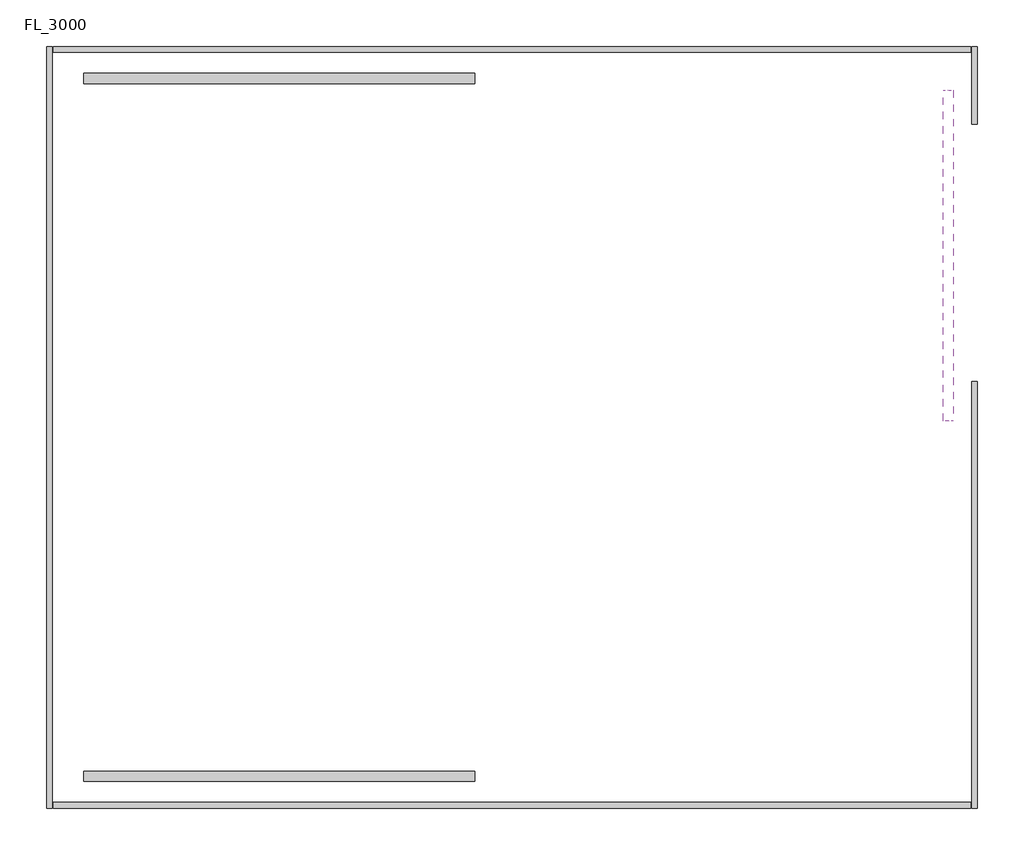
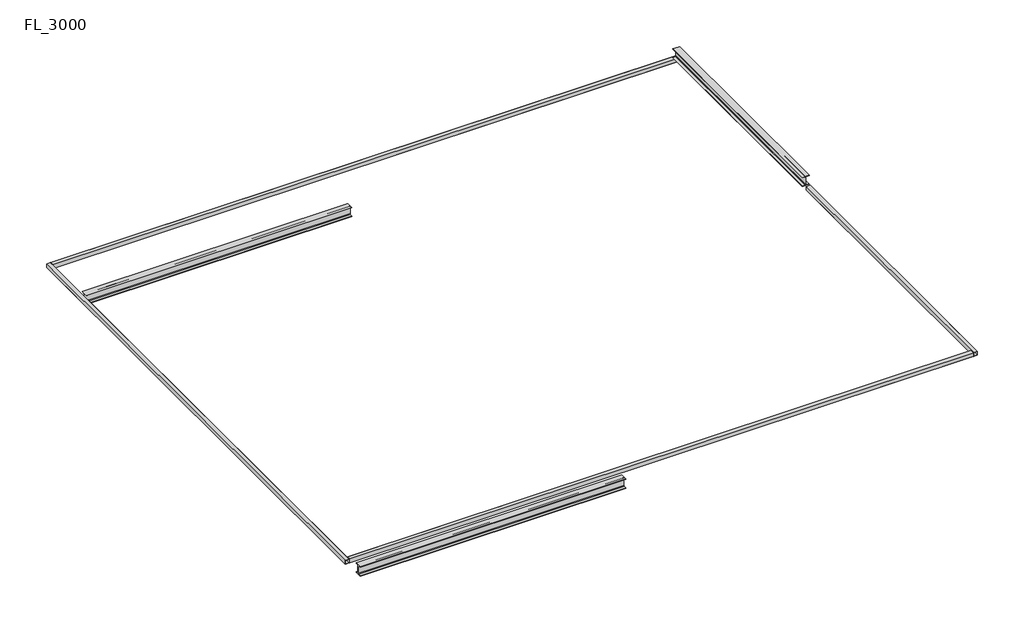
# One storey: 8 beams.
"""IFC4 building model written with IfcOpenShell, lengths in millimetres."""

import ifcopenshell
import ifcopenshell.guid

model = None  # the IFC model being written
_history = None  # IfcOwnerHistory: only IFC2X3 demands one
_inside = {}  # id of a spatial element -> (the spatial element, [elements in it])
_under = {}  # id of a project, library or spatial element -> (it, [spatial elements below it])
_declared = {}  # id of a project -> (the project, [libraries it declares])
_typed = {}  # id of a type object -> (the type object, [elements of that type])
_made_of = {}  # id of a material, layer set ... -> (it, [elements and type objects made of it])


def new_model(schema):
    """Start an empty IFC model of exactly this schema.

    Asked for "IFC4X3", IfcOpenShell would pick the latest addendum, in which some entities
    have other attributes; the version numbers below select the first issue.
    IFC2X3 requires an IfcOwnerHistory on every rooted entity: one is made here for all.
    """
    global model, _history
    if schema == "IFC4X3":
        model = ifcopenshell.file(schema_version=(4, 3, 0, 0))
    else:
        model = ifcopenshell.file(schema=schema)
    _inside.clear()
    _under.clear()
    _declared.clear()
    _typed.clear()
    _made_of.clear()
    _history = None
    if model.schema == "IFC2X3":
        org = make("IfcOrganization", Name="unknown")
        user = make(
            "IfcPersonAndOrganization",
            ThePerson=make("IfcPerson", FamilyName="unknown"),
            TheOrganization=org,
        )
        app = make(
            "IfcApplication",
            ApplicationDeveloper=org,
            Version="unknown",
            ApplicationFullName="unknown",
            ApplicationIdentifier="unknown",
        )
        _history = make(
            "IfcOwnerHistory",
            OwningUser=user,
            OwningApplication=app,
            ChangeAction="ADDED",
            CreationDate=0,
        )
    return model


def make(cls, **values):
    """One entity of the class cls with the attributes given. An attribute that is None is left unset."""
    return model.create_entity(
        cls, **{name: value for name, value in values.items() if value is not None}
    )


def rooted(cls, **values):
    """An entity with a GlobalId (a new one), such as an element, a storey or a relation."""
    return make(cls, GlobalId=ifcopenshell.guid.new(), OwnerHistory=_history, **values)


def si_unit(unit_type, name, prefix=None):
    """IfcSIUnit, for example si_unit("LENGTHUNIT", "METRE", prefix="MILLI")."""
    return make("IfcSIUnit", UnitType=unit_type, Prefix=prefix, Name=name)


def assignment(units):
    """IfcUnitAssignment: the units of a project."""
    return None if units is None else make("IfcUnitAssignment", Units=units)


def point(xyz):
    """IfcCartesianPoint."""
    return None if xyz is None else make("IfcCartesianPoint", Coordinates=xyz)


def direction(xyz):
    """IfcDirection."""
    return None if xyz is None else make("IfcDirection", DirectionRatios=xyz)


def frame(location, z_axis=None, x_axis=None):
    """IfcAxis2Placement3D, a coordinate frame: its origin and axes. An axis left out is left unset."""
    return make(
        "IfcAxis2Placement3D",
        Location=point(location),
        Axis=direction(z_axis),
        RefDirection=direction(x_axis),
    )


def frame_2d(location, x_axis=None):
    """IfcAxis2Placement2D, a coordinate frame in the plane: its origin and x axis."""
    return make(
        "IfcAxis2Placement2D", Location=point(location), RefDirection=direction(x_axis)
    )


def origin():
    """The frame at (0, 0, 0) with its axes left unset."""
    return frame((0.0, 0.0, 0.0))


def place(relative_to, where):
    """IfcLocalPlacement: puts the frame where relative to a parent placement (None: the world)."""
    return make(
        "IfcLocalPlacement", PlacementRelTo=relative_to, RelativePlacement=where
    )


def context(
    kind, dimensions, precision=None, world=None, true_north=None, identifier=None
):
    """IfcGeometricRepresentationContext, for example the 3D "Model" context."""
    return make(
        "IfcGeometricRepresentationContext",
        ContextIdentifier=identifier,
        ContextType=kind,
        CoordinateSpaceDimension=dimensions,
        Precision=precision,
        WorldCoordinateSystem=world,
        TrueNorth=true_north,
    )


def project(units=None, contexts=None):
    """IfcProject with its units and contexts."""
    return rooted(
        "IfcProject",
        Name="project",
        RepresentationContexts=contexts,
        UnitsInContext=assignment(units),
    )


def spatial(cls, under=None, at=None, **own):
    """A site, building, storey or space (cls), placed at a placement, below another one or the project."""
    s = rooted(cls, ObjectPlacement=at, **own)
    if under is not None:
        _under.setdefault(under.id(), (under, []))[1].append(s)
    return s


def polyline(points):
    """IfcPolyline through the points."""
    return make("IfcPolyline", Points=[point(p) for p in points])


def circle_curve(where, radius):
    """IfcCircle in the frame where."""
    return make("IfcCircle", Position=where, Radius=radius)


def trimmed(basis, trim1, trim2, sense, master):
    """IfcTrimmedCurve: the piece of a basis curve between two trims."""
    return make(
        "IfcTrimmedCurve",
        BasisCurve=basis,
        Trim1=trim1,
        Trim2=trim2,
        SenseAgreement=sense,
        MasterRepresentation=master,
    )


def segment(curve, same_sense, transition):
    """IfcCompositeCurveSegment."""
    return make(
        "IfcCompositeCurveSegment",
        Transition=transition,
        SameSense=same_sense,
        ParentCurve=curve,
    )


def composite_curve(segments, self_intersect=None):
    """IfcCompositeCurve: segments joined end to end."""
    return make("IfcCompositeCurve", Segments=segments, SelfIntersect=self_intersect)


def outline(outer, holes=None, kind="AREA"):
    """IfcArbitraryClosedProfileDef: a profile drawn as a closed curve; with holes, ...WithVoids."""
    if holes is None:
        return make("IfcArbitraryClosedProfileDef", ProfileType=kind, OuterCurve=outer)
    return make(
        "IfcArbitraryProfileDefWithVoids",
        ProfileType=kind,
        OuterCurve=outer,
        InnerCurves=holes,
    )


def extrude(swept, where, along, depth):
    """IfcExtrudedAreaSolid: the profile swept, set in the frame where, extruded along a direction by depth."""
    return make(
        "IfcExtrudedAreaSolid",
        SweptArea=swept,
        Position=where,
        ExtrudedDirection=direction(along),
        Depth=depth,
    )


def shape(context_of_items, identifier, shape_type, items):
    """IfcShapeRepresentation: the items that make up one representation, for example the "Body"."""
    return make(
        "IfcShapeRepresentation",
        ContextOfItems=context_of_items,
        RepresentationIdentifier=identifier,
        RepresentationType=shape_type,
        Items=items,
    )


def source(mapping_origin, context_of_items, identifier, shape_type, items):
    """IfcRepresentationMap: a shape defined once, which mapped items show again and again."""
    return make(
        "IfcRepresentationMap",
        MappingOrigin=mapping_origin,
        MappedRepresentation=shape(context_of_items, identifier, shape_type, items),
    )


def transform(
    local_origin,
    x_axis=None,
    y_axis=None,
    z_axis=None,
    scale=None,
    scale2=None,
    scale3=None,
    uniform=True,
):
    """IfcCartesianTransformationOperator3D, or its non-uniform kind. x_axis, y_axis, z_axis: its Axis1, 2, 3."""
    if uniform:
        return make(
            "IfcCartesianTransformationOperator3D",
            Axis1=direction(x_axis),
            Axis2=direction(y_axis),
            LocalOrigin=point(local_origin),
            Scale=scale,
            Axis3=direction(z_axis),
        )
    return make(
        "IfcCartesianTransformationOperator3DnonUniform",
        Axis1=direction(x_axis),
        Axis2=direction(y_axis),
        LocalOrigin=point(local_origin),
        Scale=scale,
        Axis3=direction(z_axis),
        Scale2=scale2,
        Scale3=scale3,
    )


def mapped(mapping_source, mapping_target):
    """IfcMappedItem: shows the shape of a source again, moved by a transform."""
    return make(
        "IfcMappedItem", MappingSource=mapping_source, MappingTarget=mapping_target
    )


def made_of(thing, what):
    """Note that an element or type object is made of a material, layer set ...; save() writes the relation."""
    if what is not None:
        _made_of.setdefault(what.id(), (what, []))[1].append(thing)
    return thing


def element(
    cls,
    number,
    at=None,
    inside=None,
    cuts=None,
    type_object=None,
    material=None,
    context=None,
    identifier="Body",
    shape_type=None,
    held_by="IfcProductDefinitionShape",
    body=None,
    shapes=None,
    **own,
):
    """One element of the class cls, such as IfcWall. Its Tag is "e" and its number.

    at: its placement. inside: the storey or other place that contains it. cuts: it is an
    opening in that element (IfcRelVoidsElement). A single representation is given by context,
    identifier, shape_type and body (its items); several are given by shapes. held_by: the class
    of the entity that holds the representations. save() writes the other relations.
    """
    e = rooted(cls, Tag="e%d" % number, ObjectPlacement=at, **own)
    if body is not None:
        shapes = [shape(context, identifier, shape_type, body)]
    if shapes is not None:
        e.Representation = make(held_by, Representations=shapes)
    if inside is not None:
        _inside.setdefault(inside.id(), (inside, []))[1].append(e)
    if cuts is not None:
        rooted(
            "IfcRelVoidsElement", RelatingBuildingElement=cuts, RelatedOpeningElement=e
        )
    if type_object is not None:
        _typed.setdefault(type_object.id(), (type_object, []))[1].append(e)
    return made_of(e, material)


def aggregate(whole, parts):
    """IfcRelAggregates: a whole, such as a stair, and the parts it consists of."""
    return rooted("IfcRelAggregates", RelatingObject=whole, RelatedObjects=parts)


def save(model, path):
    """Write the relations noted so far, then the file.

    IfcRelAggregates (storeys below a building ...), IfcRelContainedInSpatialStructure (elements
    in a storey), IfcRelDefinesByType, IfcRelAssociatesMaterial and IfcRelDeclares: one each for
    every whole, place, type object, material and project.
    """
    for whole, parts in _under.values():
        aggregate(whole, parts)
    for where, things in _inside.values():
        rooted(
            "IfcRelContainedInSpatialStructure",
            RelatedElements=things,
            RelatingStructure=where,
        )
    for kind, things in _typed.values():
        rooted("IfcRelDefinesByType", RelatedObjects=things, RelatingType=kind)
    for what, things in _made_of.values():
        rooted("IfcRelAssociatesMaterial", RelatedObjects=things, RelatingMaterial=what)
    for by, libraries in _declared.values():
        rooted("IfcRelDeclares", RelatingContext=by, RelatedDefinitions=libraries)
    model.write(path)


def steel_h_beam_22148b76(model_context):
    return source(origin(), model_context, "Body", "SweptSolid", [
        extrude(outline(composite_curve([segment(polyline([(87.5, -111.0), (87.5, -122.0), (-87.5, -122.0), (-87.5, -111.0), (-19.5, -111.0)]), True, "CONTINUOUS"), segment(trimmed(circle_curve(frame_2d((-19.5, -95.0)), 16.0), [point((-19.5, -111.0))], [point((-3.5, -95.0))], True, "CARTESIAN"), True, "CONTINUOUS"), segment(polyline([(-3.5, -95.0), (-3.5, 95.0)]), True, "CONTINUOUS"), segment(trimmed(circle_curve(frame_2d((-19.5, 95.0)), 16.0), [point((-3.5, 95.0))], [point((-19.5, 111.0))], True, "CARTESIAN"), True, "CONTINUOUS"), segment(polyline([(-19.5, 111.0), (-87.5, 111.0), (-87.5, 122.0), (87.5, 122.0), (87.5, 111.0), (19.5, 111.0)]), True, "CONTINUOUS"), segment(trimmed(circle_curve(frame_2d((19.5, 95.0)), 16.0), [point((19.5, 111.0))], [point((3.5, 95.0))], True, "CARTESIAN"), True, "CONTINUOUS"), segment(polyline([(3.5, 95.0), (3.5, -95.0)]), True, "CONTINUOUS"), segment(trimmed(circle_curve(frame_2d((19.5, -95.0)), 16.0), [point((3.5, -95.0))], [point((19.5, -111.0))], True, "CARTESIAN"), True, "CONTINUOUS"), segment(polyline([(19.5, -111.0), (87.5, -111.0)]), True, "CONTINUOUS")], self_intersect=False)), frame((-3361.8243373, 0.0, 0.0), z_axis=(1.0, 0.0, 0.0), x_axis=(0.0, 1.0, 0.0)), (0.0, 0.0, 1.0), 6724.6),
    ])


def steel_h_beam_0520d745(model_context):
    return source(origin(), model_context, "Body", "SweptSolid", [
        extrude(outline(composite_curve([segment(polyline([(87.5, -111.0), (87.5, -122.0), (-87.5, -122.0), (-87.5, -111.0), (-19.5, -111.0)]), True, "CONTINUOUS"), segment(trimmed(circle_curve(frame_2d((-19.5, -95.0)), 16.0), [point((-19.5, -111.0))], [point((-3.5, -95.0))], True, "CARTESIAN"), True, "CONTINUOUS"), segment(polyline([(-3.5, -95.0), (-3.5, 95.0)]), True, "CONTINUOUS"), segment(trimmed(circle_curve(frame_2d((-19.5, 95.0)), 16.0), [point((-3.5, 95.0))], [point((-19.5, 111.0))], True, "CARTESIAN"), True, "CONTINUOUS"), segment(polyline([(-19.5, 111.0), (-87.5, 111.0), (-87.5, 122.0), (87.5, 122.0), (87.5, 111.0), (19.5, 111.0)]), True, "CONTINUOUS"), segment(trimmed(circle_curve(frame_2d((19.5, 95.0)), 16.0), [point((19.5, 111.0))], [point((3.5, 95.0))], True, "CARTESIAN"), True, "CONTINUOUS"), segment(polyline([(3.5, 95.0), (3.5, -95.0)]), True, "CONTINUOUS"), segment(trimmed(circle_curve(frame_2d((19.5, -95.0)), 16.0), [point((3.5, -95.0))], [point((19.5, -111.0))], True, "CARTESIAN"), True, "CONTINUOUS"), segment(polyline([(19.5, -111.0), (87.5, -111.0)]), True, "CONTINUOUS")], self_intersect=False)), frame((-3363.2513255, 0.0, 0.0), z_axis=(1.0, 0.0, 0.0), x_axis=(0.0, 1.0, 0.0)), (0.0, 0.0, 1.0), 6724.6),
    ])


def steel_h_beam_2cee67ca(model_context):
    return source(origin(), model_context, "Body", "SweptSolid", [
        extrude(outline(composite_curve([segment(polyline([(87.5, -111.0), (87.5, -122.0), (-87.5, -122.0), (-87.5, -111.0), (-19.5, -111.0)]), True, "CONTINUOUS"), segment(trimmed(circle_curve(frame_2d((-19.5, -95.0)), 16.0), [point((-19.5, -111.0))], [point((-3.5, -95.0))], True, "CARTESIAN"), True, "CONTINUOUS"), segment(polyline([(-3.5, -95.0), (-3.5, 95.0)]), True, "CONTINUOUS"), segment(trimmed(circle_curve(frame_2d((-19.5, 95.0)), 16.0), [point((-3.5, 95.0))], [point((-19.5, 111.0))], True, "CARTESIAN"), True, "CONTINUOUS"), segment(polyline([(-19.5, 111.0), (-87.5, 111.0), (-87.5, 122.0), (87.5, 122.0), (87.5, 111.0), (19.5, 111.0)]), True, "CONTINUOUS"), segment(trimmed(circle_curve(frame_2d((19.5, 95.0)), 16.0), [point((19.5, 111.0))], [point((3.5, 95.0))], True, "CARTESIAN"), True, "CONTINUOUS"), segment(polyline([(3.5, 95.0), (3.5, -95.0)]), True, "CONTINUOUS"), segment(trimmed(circle_curve(frame_2d((19.5, -95.0)), 16.0), [point((3.5, -95.0))], [point((19.5, -111.0))], True, "CARTESIAN"), True, "CONTINUOUS"), segment(polyline([(19.5, -111.0), (87.5, -111.0)]), True, "CONTINUOUS")], self_intersect=False)), frame((-2886.3486745, 0.0, 0.0), z_axis=(1.0, 0.0, 0.0), x_axis=(0.0, 1.0, 0.0)), (0.0, 0.0, 1.0), 5681.8597388),
    ])


def steel_rectangular_beam_bm125_rt_100x100x4_0_fd47acba(model_context):
    return source(origin(), model_context, "Body", "SweptSolid", [
        extrude(outline(polyline([(-50.0, 50.0), (50.0, 50.0), (50.0, -50.0), (-50.0, -50.0), (-50.0, 50.0)]), holes=[polyline([(46.0, -46.0), (46.0, 46.0), (-46.0, 46.0), (-46.0, -46.0), (46.0, -46.0)])]), frame((-7887.3, 0.0, 0.0), z_axis=(1.0, 0.0, 0.0), x_axis=(0.0, 1.0, 0.0)), (0.0, 0.0, 1.0), 15774.6),
        extrude(outline(polyline([(-50.0, 50.0), (50.0, 50.0), (50.0, -50.0), (-50.0, -50.0), (-50.0, 50.0)]), holes=[polyline([(46.0, -46.0), (46.0, 46.0), (-46.0, 46.0), (-46.0, -46.0), (46.0, -46.0)])]), frame((-7887.3, 0.0, 0.0), z_axis=(1.0, 0.0, 0.0), x_axis=(0.0, 1.0, 0.0)), (0.0, 0.0, 1.0), 15774.6),
        extrude(outline(polyline([(-50.0, 50.0), (50.0, 50.0), (50.0, -50.0), (-50.0, -50.0), (-50.0, 50.0)]), holes=[polyline([(46.0, -46.0), (46.0, 46.0), (-46.0, 46.0), (-46.0, -46.0), (46.0, -46.0)])]), frame((-7887.3, 0.0, 0.0), z_axis=(1.0, 0.0, 0.0), x_axis=(0.0, 1.0, 0.0)), (0.0, 0.0, 1.0), 15774.6),
        extrude(outline(polyline([(-50.0, 50.0), (50.0, 50.0), (50.0, -50.0), (-50.0, -50.0), (-50.0, 50.0)]), holes=[polyline([(46.0, -46.0), (46.0, 46.0), (-46.0, 46.0), (-46.0, -46.0), (46.0, -46.0)])]), frame((-7887.3, 0.0, 0.0), z_axis=(1.0, 0.0, 0.0), x_axis=(0.0, 1.0, 0.0)), (0.0, 0.0, 1.0), 15774.6),
    ])


def steel_rectangular_beam_bm125_rt_100x100x4_0_2c93a6f0(model_context):
    return source(origin(), model_context, "Body", "SweptSolid", [
        extrude(outline(polyline([(-50.0, 50.0), (50.0, 50.0), (50.0, -50.0), (-50.0, -50.0), (-50.0, 50.0)]), holes=[polyline([(46.0, -46.0), (46.0, 46.0), (-46.0, 46.0), (-46.0, -46.0), (46.0, -46.0)])]), frame((-6550.0, 0.0, 0.0), z_axis=(1.0, 0.0, 0.0), x_axis=(0.0, 1.0, 0.0)), (0.0, 0.0, 1.0), 13100.0),
        extrude(outline(polyline([(-50.0, 50.0), (50.0, 50.0), (50.0, -50.0), (-50.0, -50.0), (-50.0, 50.0)]), holes=[polyline([(46.0, -46.0), (46.0, 46.0), (-46.0, 46.0), (-46.0, -46.0), (46.0, -46.0)])]), frame((-6550.0, 0.0, 0.0), z_axis=(1.0, 0.0, 0.0), x_axis=(0.0, 1.0, 0.0)), (0.0, 0.0, 1.0), 13100.0),
        extrude(outline(polyline([(-50.0, 50.0), (50.0, 50.0), (50.0, -50.0), (-50.0, -50.0), (-50.0, 50.0)]), holes=[polyline([(46.0, -46.0), (46.0, 46.0), (-46.0, 46.0), (-46.0, -46.0), (46.0, -46.0)])]), frame((-6550.0, 0.0, 0.0), z_axis=(1.0, 0.0, 0.0), x_axis=(0.0, 1.0, 0.0)), (0.0, 0.0, 1.0), 13100.0),
        extrude(outline(polyline([(-50.0, 50.0), (50.0, 50.0), (50.0, -50.0), (-50.0, -50.0), (-50.0, 50.0)]), holes=[polyline([(46.0, -46.0), (46.0, 46.0), (-46.0, 46.0), (-46.0, -46.0), (46.0, -46.0)])]), frame((-6550.0, 0.0, 0.0), z_axis=(1.0, 0.0, 0.0), x_axis=(0.0, 1.0, 0.0)), (0.0, 0.0, 1.0), 13100.0),
    ])


def steel_rectangular_beam_bm125_rt_100x100x4_0_bbce7aa4(model_context):
    return source(origin(), model_context, "Body", "SweptSolid", [
        extrude(outline(polyline([(-50.0, 50.0), (50.0, 50.0), (50.0, -50.0), (-50.0, -50.0), (-50.0, 50.0)]), holes=[polyline([(46.0, -46.0), (46.0, 46.0), (-46.0, 46.0), (-46.0, -46.0), (46.0, -46.0)])]), frame((-3725.0, 0.0, 0.0), z_axis=(1.0, 0.0, 0.0), x_axis=(0.0, 1.0, 0.0)), (0.0, 0.0, 1.0), 7337.3),
        extrude(outline(polyline([(-50.0, 50.0), (50.0, 50.0), (50.0, -50.0), (-50.0, -50.0), (-50.0, 50.0)]), holes=[polyline([(46.0, -46.0), (46.0, 46.0), (-46.0, 46.0), (-46.0, -46.0), (46.0, -46.0)])]), frame((-3725.0, 0.0, 0.0), z_axis=(1.0, 0.0, 0.0), x_axis=(0.0, 1.0, 0.0)), (0.0, 0.0, 1.0), 7337.3),
        extrude(outline(polyline([(-50.0, 50.0), (50.0, 50.0), (50.0, -50.0), (-50.0, -50.0), (-50.0, 50.0)]), holes=[polyline([(46.0, -46.0), (46.0, 46.0), (-46.0, 46.0), (-46.0, -46.0), (46.0, -46.0)])]), frame((-3725.0, 0.0, 0.0), z_axis=(1.0, 0.0, 0.0), x_axis=(0.0, 1.0, 0.0)), (0.0, 0.0, 1.0), 7337.3),
        extrude(outline(polyline([(-50.0, 50.0), (50.0, 50.0), (50.0, -50.0), (-50.0, -50.0), (-50.0, 50.0)]), holes=[polyline([(46.0, -46.0), (46.0, 46.0), (-46.0, 46.0), (-46.0, -46.0), (46.0, -46.0)])]), frame((-3725.0, 0.0, 0.0), z_axis=(1.0, 0.0, 0.0), x_axis=(0.0, 1.0, 0.0)), (0.0, 0.0, 1.0), 7337.3),
    ])


def steel_rectangular_beam_bm125_rt_100x100x4_0_d4cde651(model_context):
    return source(origin(), model_context, "Body", "SweptSolid", [
        extrude(outline(polyline([(-50.0, 50.0), (50.0, 50.0), (50.0, -50.0), (-50.0, -50.0), (-50.0, 50.0)]), holes=[polyline([(46.0, -46.0), (46.0, 46.0), (-46.0, 46.0), (-46.0, -46.0), (46.0, -46.0)])]), frame((-612.3, 0.0, 0.0), z_axis=(1.0, 0.0, 0.0), x_axis=(0.0, 1.0, 0.0)), (0.0, 0.0, 1.0), 1337.3),
        extrude(outline(polyline([(-50.0, 50.0), (50.0, 50.0), (50.0, -50.0), (-50.0, -50.0), (-50.0, 50.0)]), holes=[polyline([(46.0, -46.0), (46.0, 46.0), (-46.0, 46.0), (-46.0, -46.0), (46.0, -46.0)])]), frame((-612.3, 0.0, 0.0), z_axis=(1.0, 0.0, 0.0), x_axis=(0.0, 1.0, 0.0)), (0.0, 0.0, 1.0), 1337.3),
        extrude(outline(polyline([(-50.0, 50.0), (50.0, 50.0), (50.0, -50.0), (-50.0, -50.0), (-50.0, 50.0)]), holes=[polyline([(46.0, -46.0), (46.0, 46.0), (-46.0, 46.0), (-46.0, -46.0), (46.0, -46.0)])]), frame((-612.3, 0.0, 0.0), z_axis=(1.0, 0.0, 0.0), x_axis=(0.0, 1.0, 0.0)), (0.0, 0.0, 1.0), 1337.3),
        extrude(outline(polyline([(-50.0, 50.0), (50.0, 50.0), (50.0, -50.0), (-50.0, -50.0), (-50.0, 50.0)]), holes=[polyline([(46.0, -46.0), (46.0, 46.0), (-46.0, 46.0), (-46.0, -46.0), (46.0, -46.0)])]), frame((-612.3, 0.0, 0.0), z_axis=(1.0, 0.0, 0.0), x_axis=(0.0, 1.0, 0.0)), (0.0, 0.0, 1.0), 1337.3),
    ])


model = new_model("IFC4")

# Units and contexts
model_context = context("Model", 3, world=origin())
ifc_project = project(units=[si_unit("LENGTHUNIT", "METRE", prefix="MILLI")], contexts=[model_context])

# Site, building, storey
site = spatial("IfcSite", under=ifc_project)
building = spatial("IfcBuilding", under=site)
storey = spatial("IfcBuildingStorey", under=building, Name="FL_3000", Elevation=3000.0)

# Beams
placement = place(None, origin())
steel_h_beam_shape = steel_h_beam_22148b76(model_context)
element("IfcBeam", 1, ObjectType="Steel-H-Beam : BM121_H-244×175x7x11", at=placement, inside=storey, context=model_context, shape_type="MappedRepresentation", body=[
    mapped(steel_h_beam_shape, transform((2100.4756627, 10594.5382614, 3000.0), x_axis=(1.0, 0.0, 0.0), y_axis=(0.0, 1.0, 0.0), z_axis=(0.0, 0.0, 1.0))),
])
steel_h_beam_2_shape = steel_h_beam_0520d745(model_context)
element("IfcBeam", 2, ObjectType="Steel-H-Beam : BM121_H-244×175x7x11", at=placement, inside=storey, context=model_context, shape_type="MappedRepresentation", body=[
    mapped(steel_h_beam_2_shape, transform((2100.0, 22594.5382614, 3000.0), x_axis=(-1.0, 0.0, 0.0), y_axis=(0.0, -1.0, 0.0), z_axis=(0.0, 0.0, 1.0))),
])
steel_h_beam_3_shape = steel_h_beam_2cee67ca(model_context)
element("IfcBeam", 3, ObjectType="Steel-H-Beam : BM121_H-244×175x7x11", at=placement, inside=storey, context=model_context, shape_type="MappedRepresentation", body=[
    mapped(steel_h_beam_3_shape, transform((13600.0, 19594.5382614, 4500.0), x_axis=(0.0, 1.0, 0.0), y_axis=(-1.0, 0.0, 0.0), z_axis=(0.0, 0.0, 1.0))),
])
steel_rectangular_beam_bm125_rt_100x100x4_0_shape = steel_rectangular_beam_bm125_rt_100x100x4_0_fd47acba(model_context)
element("IfcBeam", 4, ObjectType="Steel-Rectangular-Beam : BM125_RT-100x100x4.0", at=placement, inside=storey, context=model_context, shape_type="MappedRepresentation", body=[
    mapped(steel_rectangular_beam_bm125_rt_100x100x4_0_shape, transform((6100.0, 10094.5382614, 3750.0), x_axis=(1.0, 0.0, 0.0), y_axis=(0.0, 1.0, 0.0), z_axis=(0.0, 0.0, 1.0))),
])
element("IfcBeam", 5, ObjectType="Steel-Rectangular-Beam : BM125_RT-100x100x4.0", at=placement, inside=storey, context=model_context, shape_type="MappedRepresentation", body=[
    mapped(steel_rectangular_beam_bm125_rt_100x100x4_0_shape, transform((6100.0, 23094.5382614, 3750.0), x_axis=(-1.0, 0.0, 0.0), y_axis=(0.0, -1.0, 0.0), z_axis=(0.0, 0.0, 1.0))),
])
steel_rectangular_beam_bm125_rt_100x100x4_0_2_shape = steel_rectangular_beam_bm125_rt_100x100x4_0_2c93a6f0(model_context)
element("IfcBeam", 6, ObjectType="Steel-Rectangular-Beam : BM125_RT-100x100x4.0", at=placement, inside=storey, context=model_context, shape_type="MappedRepresentation", body=[
    mapped(steel_rectangular_beam_bm125_rt_100x100x4_0_2_shape, transform((-1850.0, 16594.5382614, 3750.0), x_axis=(0.0, -1.0, 0.0), y_axis=(1.0, 0.0, 0.0), z_axis=(0.0, 0.0, 1.0))),
])
steel_rectangular_beam_bm125_rt_100x100x4_0_3_shape = steel_rectangular_beam_bm125_rt_100x100x4_0_bbce7aa4(model_context)
element("IfcBeam", 7, ObjectType="Steel-Rectangular-Beam : BM125_RT-100x100x4.0", at=placement, inside=storey, context=model_context, shape_type="MappedRepresentation", body=[
    mapped(steel_rectangular_beam_bm125_rt_100x100x4_0_3_shape, transform((14050.0, 13769.5382614, 3750.0), x_axis=(0.0, 1.0, 0.0), y_axis=(-1.0, 0.0, 0.0), z_axis=(0.0, 0.0, 1.0))),
])
steel_rectangular_beam_bm125_rt_100x100x4_0_4_shape = steel_rectangular_beam_bm125_rt_100x100x4_0_d4cde651(model_context)
element("IfcBeam", 8, ObjectType="Steel-Rectangular-Beam : BM125_RT-100x100x4.0", at=placement, inside=storey, context=model_context, shape_type="MappedRepresentation", body=[
    mapped(steel_rectangular_beam_bm125_rt_100x100x4_0_4_shape, transform((14050.0, 22419.5382614, 3750.0), x_axis=(0.0, 1.0, 0.0), y_axis=(-1.0, 0.0, 0.0), z_axis=(0.0, 0.0, 1.0))),
])

save(model, "model.ifc")

# Revit data of these elements
# Type "Steel-H-Beam : BM121_H-244×175x7x11"
#   Surface Area = 1.14653 m²/m
#   Section Area = 56.2375 cm²
#   Mass per Unit Length = 44.1465 kg/m
#   Length [instance default] = 3000 mm
#   B = 175 mm
#   H = 244 mm
#   r = 16 mm
#   tw = 7 mm
#   tf = 11 mm
#   hec_material4 [instance default] = none
#   hec_material3 [instance default] = none
#   hec_material2 [instance default] = none
#   hec_material1 [instance default] = none
#   Structural Material [instance default] = Steel, 45-345
#   Assembly Code = ""
# Type "Steel-Rectangular-Beam : BM125_RT-100x100x4.0"
#   t = 4 mm
#   Mass per Unit Length = 11.70 kg/m
#   Surface Area = 0.386 m²/m
#   Sectional Area = 14.95 cm²
#   Length [instance default] = 3000 mm
#   H = 100 mm
#   B = 100 mm
#   hec_material4 [instance default] = none
#   hec_material3 [instance default] = none
#   hec_material2 [instance default] = none
#   hec_material1 [instance default] = none
#   Structural Material [instance default] = none
# Elements 1, 2, 3 (IfcBeam, "Steel-H-Beam : BM121_H-244×175x7x11")
#   Comments = ""
#   F01) Building Name = "Fire Water Pump Building"
#   F11) Project Building Tag_Type-1 = ""
#   F12) Project Building Tag_Type-2 = ""
#   F13) Project Facility Code = "621"
#   F21) Structural Type = "Steel"
#   F31) Standard Building Code = "E204"
#   F41) Discipline = "Architecture"
#   F51) Plan Start Date-Engineering = "2018-09-14"
#   F52) Plan Finish Date-Engineering = "2019-12-02"
#   F53) Duration = "444"
#   W11) Activity ID = "T3C621AR4110"
#   W12) Activity Name = "Fire Water Pump BLDG - Main Steel Structure"
#   W13) Plan Start Date = "2019-04-02"
#   W14) Plan Finish Date = "2019-06-03"
#   Structural Material = S01AA002-00001_Main Steel Structure Fabrication Work_Shelter/Building_Medium Steel - Standard
#   hec_material4 = none
#   hec_material3 = none
#   hec_material2 = F01AC000-00002_Building/Shelter Fire Proofing Work_Intumescent Coating Type_1 hr. rating (UL 1709))
#   hec_material1 = S01AA010-00002_Main Steel Structure Fabrication Work_Shelter/Building_Steel Painting/Coating_for Fireproofed Steel Surface, Surface Preparation & Primer Coat
#   Structural Material = S03AA028-00001_Main Steel Structure Erection Work_Shelter/Building_Medium Steel
#   Phase Created = New Construction
#   Materials on its faces: "S03AA028-00001_Main Steel Structure Erection Work_Shelter/Building_Medium Steel"
# Elements 4, 5, 6, 7, 8 (IfcBeam, "Steel-Rectangular-Beam : BM125_RT-100x100x4.0")
#   Comments = ""
#   F01) Building Name = "Fire Water Pump Building"
#   F11) Project Building Tag_Type-1 = ""
#   F12) Project Building Tag_Type-2 = ""
#   F13) Project Facility Code = "621"
#   F21) Structural Type = "Steel"
#   F31) Standard Building Code = "E204"
#   F41) Discipline = "Architecture"
#   F51) Plan Start Date-Engineering = "2018-09-14"
#   F52) Plan Finish Date-Engineering = "2019-12-02"
#   F53) Duration = "444"
#   W11) Activity ID = "T3C621AR4110"
#   W12) Activity Name = "Fire Water Pump BLDG - Main Steel Structure"
#   W13) Plan Start Date = "2019-04-02"
#   W14) Plan Finish Date = "2019-06-03"
#   hec_material4 = none
#   hec_material3 = none
#   hec_material2 = S01AA010-00001_Main Steel Structure Fabrication Work_Shelter/Building_Steel Painting/Coating_for Non-Fireproofed Steel Surface, Surface Preparation, Primer, Second & Final Coat
#   hec_material1 = S03AA007-00001_Main Steel Structure Erection Work_Girth & Purlin
#   Structural Material = S01AA007-00001_Main Steel Structure Fabrication Work_Shelter/Building_Girth & Purlin
#   Phase Created = New Construction
#   Materials on its faces: "S01AA010-00001_Main Steel Structure Fabrication Work_Shelter/Building_Steel Painting/Coating_for Non-Fireproofed Steel Surface, Surface Preparation, Primer, Second & Final Coat"
# Materials
#   "Steel, 45-345": class "Metal", colour RGB 189 187 185, transparency 0, Description = "Steel 345 MPa", Cost = 0
#   "S03AA028-00001_Main Steel Structure Erection Work_Shelter/Building_Medium Steel": class "Metal", colour RGB 120 120 120, transparency 0, Comments = "(90KG/M>Weight≥30KG/M)", Description = "Structural steel 50ksi", W00) Work Master Code = "S03AA028-0001", W01) Work Master_Lv1 = "Main Steel Structure Erection Work", W02) Work Master_Lv2 = "Shelter/Building", W03) Work Master_Spec.1 = "Medium Steel (90KG/M>Weight≥30KG/M)", Cost = 0
#   "S01AA002-00001_Main Steel Structure Fabrication Work_Shelter/Building_Medium Steel - Standard": class "Metal", colour RGB 120 120 120, transparency 0, Comments = "(90KG/M>Weight≥30KG/M)", Description = "Structural steel 50ksi", W00) Work Master Code = "S01AA002-0001", W01) Work Master_Lv1 = "Main Steel Structure Fabrication Work", W02) Work Master_Lv2 = "Shelter/Building", W03) Work Master_Spec.1 = "Medium Steel - Standard (90KG/M>Weight≥30KG/M)", Cost = 0
#   "F01AC000-00002_Building/Shelter Fire Proofing Work_Intumescent Coating Type_1 hr. rating (UL 1709))": class "Metal", colour RGB 255 128 128, transparency 0, Description = "Paint finished steel", W00) Work Master Code = "F01AC000-00002", W01) Work Master_Lv1 = "Building/Shelter Fire Proofing Work", W02) Work Master_Lv2 = "Intumescent Coating Type", W03) Work Master_Spec.1 = "1 hr. rating (UL 1709)", Cost = 0
#   "S01AA010-00002_Main Steel Structure Fabrication Work_Shelter/Building_Steel Painting/Coating_for Fireproofed Steel Surface, Surface Preparation & Primer Coat": class "Metal", colour RGB 120 120 120, transparency 0, Description = "Paint finished steel", W00) Work Master Code = "SS01AA010-00002", W01) Work Master_Lv1 = "Main Steel Structure Fabrication Work", W02) Work Master_Lv2 = "Shelter/Building", W03) Work Master_Spec.1 = "Steel Painting/Coating", W04) Work Master_Spec.2 = "for Fireproofed Steel Surface, Surface Preparation & Primer Coat", Cost = 0
#   "S01AA010-00001_Main Steel Structure Fabrication Work_Shelter/Building_Steel Painting/Coating_for Non-Fireproofed Steel Surface, Surface Preparation, Primer, Second & Final Coat": class "Metal", colour RGB 120 120 120, transparency 0, Description = "Paint finished steel", W00) Work Master Code = "S01AA010-00001", W01) Work Master_Lv1 = "Main Steel Structure Fabrication Work", W02) Work Master_Lv2 = "Shelter/Building", W03) Work Master_Spec.1 = "Steel Painting/Coating", W04) Work Master_Spec.2 = "for Non-Fireproofed Steel Surface, Surface Preparation, Primer, Second & Final Coat", Cost = 0
#   "S03AA007-00001_Main Steel Structure Erection Work_Girth & Purlin": class "Metal", colour RGB 120 120 120, transparency 0, Comments = "(30KG/M>Weight)", Description = "Structural steel 50ksi", W00) Work Master Code = "S03AA007-00001", W01) Work Master_Lv1 = "Main Steel Structure Erection Work", W02) Work Master_Lv2 = "Shelter/Building", W03) Work Master_Spec.1 = "Girth & Purlin", Cost = 0
#   "S01AA007-00001_Main Steel Structure Fabrication Work_Shelter/Building_Girth & Purlin": class "Metal", colour RGB 120 120 120, transparency 0, Comments = "(30KG/M>Weight)", Description = "Structural steel 50ksi", W00) Work Master Code = "S01AA007-00001", W01) Work Master_Lv1 = "Main Steel Structure Fabrication Work", W02) Work Master_Lv2 = "Shelter/Building", W03) Work Master_Spec.1 = "Girth & Purlin", Cost = 0
